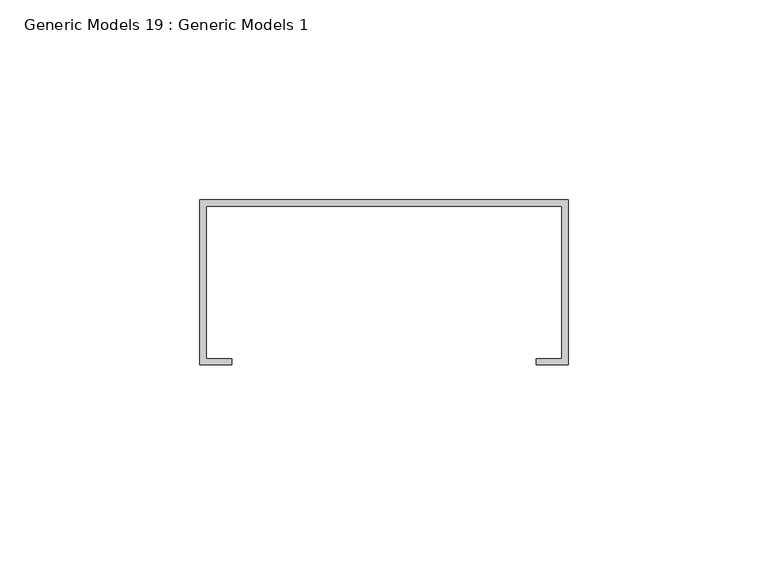
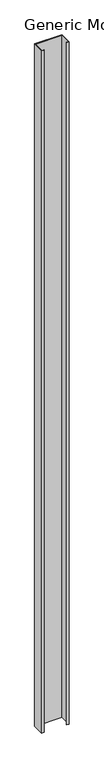
"""IFC4 building model written with IfcOpenShell, lengths in millimetres: proxy geometry, Generic Models 19 : Generic Models 1."""

from ifc_helpers import new_model, si_unit, frame, origin, place, context, project, spatial, polyline, outline, extrude, source, transform, mapped, element, save


def generic_models_19_generic_models_1_274f06fa(model_context):
    return source(origin(), model_context, "Body", "SweptSolid", [
        extrude(outline(polyline([(49691.925, 630.2375), (49784.0, 630.2375), (49784.0, 588.9625), (49776.0625, 588.9625), (49776.0625, 590.55), (49782.4125, 590.55), (49782.4125, 628.65), (49693.5125, 628.65), (49693.5125, 590.55), (49699.8625, 590.55), (49699.8625, 588.9625), (49691.925, 588.9625), (49691.925, 630.2375)])), frame((0.0, 0.0, 1.5875), z_axis=(0.0, 0.0, 1.0), x_axis=(1.0, 0.0, 0.0)), (0.0, 0.0, 1.0), 2428.875),
    ])


if __name__ == "__main__":
    model = new_model("IFC4")
    model_context = context("Model", 3, world=origin())
    ifc_project = project(units=[si_unit("LENGTHUNIT", "METRE", prefix="MILLI")], contexts=[model_context])
    site = spatial("IfcSite", under=ifc_project)
    building = spatial("IfcBuilding", under=site)
    placement = place(None, origin())
    generic_models_19_generic_models_1_shape = generic_models_19_generic_models_1_274f06fa(model_context)
    element("IfcBuildingElementProxy", 1, Name="Generic Models 19 : Generic Models 1", ObjectType="Generic Models 19 : Generic Models 1", at=placement, inside=building, context=model_context, shape_type="MappedRepresentation", body=[
        mapped(generic_models_19_generic_models_1_shape, transform((0.0, 0.0, 0.0), x_axis=(1.0, 0.0, 0.0), y_axis=(0.0, 1.0, 0.0), z_axis=(0.0, 0.0, 1.0))),
    ])
    save(model, "model.ifc")

# Revit data of these elements
# Element 1 (IfcBuildingElementProxy, "Generic Models 19 : Generic Models 1")
#   Materials on its faces: "METAL STUDS (MATCH EXISTING SIZE/GAUGE/SPACING)"
# Materials
#   "METAL STUDS (MATCH EXISTING SIZE/GAUGE/SPACING)": class "Unassigned", colour RGB 210 209 208, transparency 0, Keynote = "M05121300.02", Cost = 0
